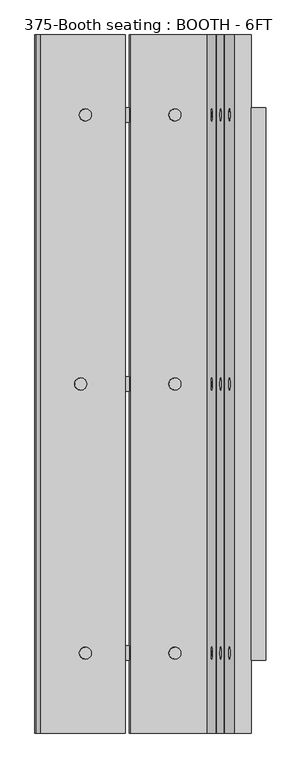
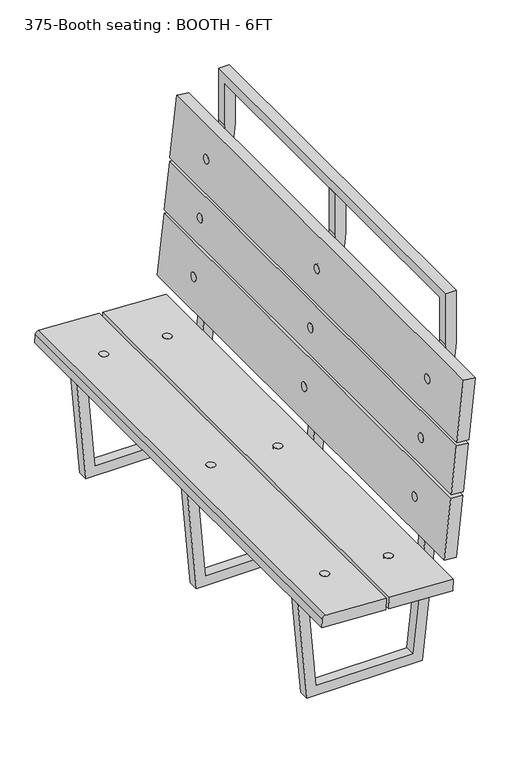
"""IFC4 building model written with IfcOpenShell, lengths in millimetres: furniture geometry, 375-Booth seating : BOOTH - 6FT."""

from ifc_helpers import new_model, si_unit, point, frame, frame_2d, origin, place, context, project, spatial, polyline, circle_curve, trimmed, segment, composite_curve, outline, extrude, faceted_brep, source, transform, mapped, element, save


def furniture_375_booth_seating_booth_6ft_eb83aa60(model_context):
    return source(origin(), model_context, "Body", "SolidModel", [
        extrude(outline(composite_curve([segment(trimmed(circle_curve(frame_2d((0.0, -15.875)), 15.875), [point((0.0, -31.75))], [point((0.0, 0.0))], False, "CARTESIAN"), True, "CONTINUOUS"), segment(trimmed(circle_curve(frame_2d((0.0, -15.875)), 15.875), [point((0.0, 0.0))], [point((0.0, -31.75))], False, "CARTESIAN"), True, "CONTINUOUS")], self_intersect=False)), frame((476.8022404, 688.975, 403.0070028), z_axis=(0.052335956242943765, 0.0, 0.9986295347545739), x_axis=(-0.9986295347545739, 0.0, 0.052335956242943765)), (0.0, 0.0, 1.0), 44.45),
        extrude(outline(composite_curve([segment(trimmed(circle_curve(frame_2d((-234.95, -15.875)), 15.875), [point((-234.95, -31.75))], [point((-234.95, 0.0))], False, "CARTESIAN"), True, "CONTINUOUS"), segment(trimmed(circle_curve(frame_2d((-234.95, -15.875)), 15.875), [point((-234.95, 0.0))], [point((-234.95, -31.75))], False, "CARTESIAN"), True, "CONTINUOUS")], self_intersect=False)), frame((476.8022404, 688.975, 403.0070028), z_axis=(0.052335956242943765, 0.0, 0.9986295347545739), x_axis=(-0.9986295347545739, 0.0, 0.052335956242943765)), (0.0, 0.0, 1.0), 44.45),
        extrude(outline(composite_curve([segment(trimmed(circle_curve(frame_2d((0.0, 1393.825)), 15.875), [point((0.0, 1377.95))], [point((0.0, 1409.7))], False, "CARTESIAN"), True, "CONTINUOUS"), segment(trimmed(circle_curve(frame_2d((0.0, 1393.825)), 15.875), [point((0.0, 1409.7))], [point((0.0, 1377.95))], False, "CARTESIAN"), True, "CONTINUOUS")], self_intersect=False)), frame((476.8022404, 688.975, 403.0070028), z_axis=(0.052335956242943765, 0.0, 0.9986295347545739), x_axis=(-0.9986295347545739, 0.0, 0.052335956242943765)), (0.0, 0.0, 1.0), 44.45),
        extrude(outline(composite_curve([segment(trimmed(circle_curve(frame_2d((-234.95, 1393.825)), 15.875), [point((-234.95, 1377.95))], [point((-234.95, 1409.7))], False, "CARTESIAN"), True, "CONTINUOUS"), segment(trimmed(circle_curve(frame_2d((-234.95, 1393.825)), 15.875), [point((-234.95, 1409.7))], [point((-234.95, 1377.95))], False, "CARTESIAN"), True, "CONTINUOUS")], self_intersect=False)), frame((476.8022404, 688.975, 403.0070028), z_axis=(0.052335956242943765, 0.0, 0.9986295347545739), x_axis=(-0.9986295347545739, 0.0, 0.052335956242943765)), (0.0, 0.0, 1.0), 44.45),
        extrude(outline(composite_curve([segment(trimmed(circle_curve(frame_2d((0.0, -15.875)), 15.875), [point((0.0, -31.75))], [point((0.0, 0.0))], False, "CARTESIAN"), True, "CONTINUOUS"), segment(trimmed(circle_curve(frame_2d((0.0, -15.875)), 15.875), [point((0.0, 0.0))], [point((0.0, -31.75))], False, "CARTESIAN"), True, "CONTINUOUS")], self_intersect=False)), frame((900.6975371, -720.725, 1069.1522612), z_axis=(-0.9945218953682735, 0.0, 0.10452846326765225), x_axis=(-0.10452846326765225, 0.0, -0.9945218953682735)), (0.0, 0.0, 1.0), 44.45),
        extrude(outline(composite_curve([segment(trimmed(circle_curve(frame_2d((222.2499999, -15.875)), 15.875), [point((222.2499999, -31.75))], [point((222.2499999, 0.0))], False, "CARTESIAN"), True, "CONTINUOUS"), segment(trimmed(circle_curve(frame_2d((222.2499999, -15.875)), 15.875), [point((222.2499999, 0.0))], [point((222.2499999, -31.75))], False, "CARTESIAN"), True, "CONTINUOUS")], self_intersect=False)), frame((900.6975371, -720.725, 1069.1522612), z_axis=(-0.9945218953682735, 0.0, 0.10452846326765225), x_axis=(-0.10452846326765225, 0.0, -0.9945218953682735)), (0.0, 0.0, 1.0), 44.45),
        extrude(outline(composite_curve([segment(trimmed(circle_curve(frame_2d((444.5, -15.875)), 15.875), [point((444.5, -31.75))], [point((444.5, 0.0))], False, "CARTESIAN"), True, "CONTINUOUS"), segment(trimmed(circle_curve(frame_2d((444.5, -15.875)), 15.875), [point((444.5, 0.0))], [point((444.5, -31.75))], False, "CARTESIAN"), True, "CONTINUOUS")], self_intersect=False)), frame((900.6975371, -720.725, 1069.1522612), z_axis=(-0.9945218953682735, 0.0, 0.10452846326765225), x_axis=(-0.10452846326765225, 0.0, -0.9945218953682735)), (0.0, 0.0, 1.0), 44.45),
        extrude(outline(composite_curve([segment(trimmed(circle_curve(frame_2d((0.0, -1425.575)), 15.875), [point((0.0, -1441.45))], [point((0.0, -1409.7))], False, "CARTESIAN"), True, "CONTINUOUS"), segment(trimmed(circle_curve(frame_2d((0.0, -1425.575)), 15.875), [point((0.0, -1409.7))], [point((0.0, -1441.45))], False, "CARTESIAN"), True, "CONTINUOUS")], self_intersect=False)), frame((900.6975371, -720.725, 1069.1522612), z_axis=(-0.9945218953682735, 0.0, 0.10452846326765225), x_axis=(-0.10452846326765225, 0.0, -0.9945218953682735)), (0.0, 0.0, 1.0), 44.45),
        extrude(outline(composite_curve([segment(trimmed(circle_curve(frame_2d((222.2499999, -1425.575)), 15.875), [point((222.2499999, -1441.45))], [point((222.2499999, -1409.7))], False, "CARTESIAN"), True, "CONTINUOUS"), segment(trimmed(circle_curve(frame_2d((222.2499999, -1425.575)), 15.875), [point((222.2499999, -1409.7))], [point((222.2499999, -1441.45))], False, "CARTESIAN"), True, "CONTINUOUS")], self_intersect=False)), frame((900.6975371, -720.725, 1069.1522612), z_axis=(-0.9945218953682735, 0.0, 0.10452846326765225), x_axis=(-0.10452846326765225, 0.0, -0.9945218953682735)), (0.0, 0.0, 1.0), 44.45),
        extrude(outline(composite_curve([segment(trimmed(circle_curve(frame_2d((444.5, -1425.575)), 15.875), [point((444.5, -1441.45))], [point((444.5, -1409.7))], False, "CARTESIAN"), True, "CONTINUOUS"), segment(trimmed(circle_curve(frame_2d((444.5, -1425.575)), 15.875), [point((444.5, -1409.7))], [point((444.5, -1441.45))], False, "CARTESIAN"), True, "CONTINUOUS")], self_intersect=False)), frame((900.6975371, -720.725, 1069.1522612), z_axis=(-0.9945218953682735, 0.0, 0.10452846326765225), x_axis=(-0.10452846326765225, 0.0, -0.9945218953682735)), (0.0, 0.0, 1.0), 44.45),
        extrude(outline(composite_curve([segment(trimmed(circle_curve(frame_2d((0.0, -15.875)), 15.875), [point((0.0, -31.75))], [point((0.0, 0.0))], False, "CARTESIAN"), True, "CONTINUOUS"), segment(trimmed(circle_curve(frame_2d((0.0, -15.875)), 15.875), [point((0.0, 0.0))], [point((0.0, -31.75))], False, "CARTESIAN"), True, "CONTINUOUS")], self_intersect=False)), frame((464.1196453, -15.875, 403.6716695), z_axis=(0.052335956242943765, 0.0, 0.9986295347545739), x_axis=(-0.9986295347545739, 0.0, 0.052335956242943765)), (0.0, 0.0, 1.0), 44.45),
        extrude(outline(composite_curve([segment(trimmed(circle_curve(frame_2d((-247.65, -15.875)), 15.875), [point((-247.65, -31.75))], [point((-247.65, 0.0))], False, "CARTESIAN"), True, "CONTINUOUS"), segment(trimmed(circle_curve(frame_2d((-247.65, -15.875)), 15.875), [point((-247.65, 0.0))], [point((-247.65, -31.75))], False, "CARTESIAN"), True, "CONTINUOUS")], self_intersect=False)), frame((464.1196453, -15.875, 403.6716695), z_axis=(0.052335956242943765, 0.0, 0.9986295347545739), x_axis=(-0.9986295347545739, 0.0, 0.052335956242943765)), (0.0, 0.0, 1.0), 44.45),
        extrude(outline(composite_curve([segment(trimmed(circle_curve(frame_2d((0.0, -15.875)), 15.875), [point((0.0, -31.75))], [point((0.0, 0.0))], False, "CARTESIAN"), True, "CONTINUOUS"), segment(trimmed(circle_curve(frame_2d((0.0, -15.875)), 15.875), [point((0.0, 0.0))], [point((0.0, -31.75))], False, "CARTESIAN"), True, "CONTINUOUS")], self_intersect=False)), frame((900.6975371, -15.875, 1069.1522612), z_axis=(-0.9945218953682735, 0.0, 0.10452846326765225), x_axis=(-0.10452846326765225, 0.0, -0.9945218953682735)), (0.0, 0.0, 1.0), 44.45),
        extrude(outline(composite_curve([segment(trimmed(circle_curve(frame_2d((222.2499999, -15.875)), 15.875), [point((222.2499999, -31.75))], [point((222.2499999, 0.0))], False, "CARTESIAN"), True, "CONTINUOUS"), segment(trimmed(circle_curve(frame_2d((222.2499999, -15.875)), 15.875), [point((222.2499999, 0.0))], [point((222.2499999, -31.75))], False, "CARTESIAN"), True, "CONTINUOUS")], self_intersect=False)), frame((900.6975371, -15.875, 1069.1522612), z_axis=(-0.9945218953682735, 0.0, 0.10452846326765225), x_axis=(-0.10452846326765225, 0.0, -0.9945218953682735)), (0.0, 0.0, 1.0), 44.45),
        extrude(outline(composite_curve([segment(trimmed(circle_curve(frame_2d((444.5, -15.875)), 15.875), [point((444.5, -31.75))], [point((444.5, 0.0))], False, "CARTESIAN"), True, "CONTINUOUS"), segment(trimmed(circle_curve(frame_2d((444.5, -15.875)), 15.875), [point((444.5, 0.0))], [point((444.5, -31.75))], False, "CARTESIAN"), True, "CONTINUOUS")], self_intersect=False)), frame((900.6975371, -15.875, 1069.1522612), z_axis=(-0.9945218953682735, 0.0, 0.10452846326765225), x_axis=(-0.10452846326765225, 0.0, -0.9945218953682735)), (0.0, 0.0, 1.0), 44.45),
        extrude(outline(polyline([(384.5625035, 828.7442542), (408.7701083, 366.8356381), (0.0, 402.5983885), (0.0, 826.6349718), (1193.8, 952.1084079), (1358.9, 952.1084079), (1358.9, 914.0084079), (1195.7967364, 914.0084079), (384.5625035, 828.7442542)]), holes=[polyline([(38.1, 437.5106063), (368.4284885, 408.6106083), (346.6192193, 824.7562543), (38.1, 792.3295777), (38.1, 437.5106063)])]), frame((0.0, -19.05, 0.0), z_axis=(0.0, 1.0, 0.0), x_axis=(0.0, 0.0, 1.0)), (0.0, 0.0, 1.0), 38.1),
        faceted_brep([(828.7442542, -685.8, 384.5625035), (914.0084079, -685.8, 1195.7967364), (914.0084079, -685.8, 1358.9), (952.1084079, -685.8, 1358.9), (952.1084079, -685.8, 1193.8), (826.6349718, -685.8, 0.0), (402.5983885, -685.8, 0.0), (366.8356381, -685.8, 408.7701083), (437.5106063, -685.8, 38.1), (792.3295777, -685.8, 38.1), (824.7562543, -685.8, 346.6192193), (408.6106083, -685.8, 368.4284885), (828.7442542, -723.9, 384.5625035), (366.8356381, -723.9, 408.7701083), (402.5983885, -723.9, 0.0), (826.6349718, -723.9, 0.0), (952.1084079, -723.9, 1193.8), (952.1084079, -723.9, 1397.0), (914.0084079, -723.9, 1397.0), (914.0084079, -723.9, 1195.7967364), (437.5106063, -723.9, 38.1), (408.6106083, -723.9, 368.4284885), (824.7562543, -723.9, 346.6192193), (792.3295777, -723.9, 38.1), (914.0084079, 685.8, 1358.9), (952.1084079, 685.8, 1358.9), (828.7442542, 723.9, 384.5625035), (914.0084079, 723.9, 1195.7967364), (914.0084079, 723.9, 1397.0), (952.1084079, 723.9, 1397.0), (952.1084079, 723.9, 1193.8), (826.6349718, 723.9, 0.0), (402.5983885, 723.9, 0.0), (366.8356381, 723.9, 408.7701083), (437.5106063, 723.9, 38.1), (792.3295777, 723.9, 38.1), (824.7562543, 723.9, 346.6192193), (408.6106083, 723.9, 368.4284885), (828.7442542, 685.8, 384.5625035), (366.8356381, 685.8, 408.7701083), (402.5983885, 685.8, 0.0), (826.6349718, 685.8, 0.0), (952.1084079, 685.8, 1193.8), (914.0084079, 685.8, 1195.7967364), (437.5106063, 685.8, 38.1), (408.6106083, 685.8, 368.4284885), (824.7562543, 685.8, 346.6192193), (792.3295777, 685.8, 38.1)], [[[0, 1, 2, 3, 4, 5, 6, 7], [8, 9, 10, 11]], [[12, 13, 14, 15, 16, 17, 18, 19], [20, 21, 22, 23]], [[5, 4, 16, 15]], [[1, 0, 12, 19]], [[0, 7, 13, 12]], [[7, 6, 14, 13]], [[6, 5, 15, 14]], [[8, 11, 21, 20]], [[11, 10, 22, 21]], [[10, 9, 23, 22]], [[9, 8, 20, 23]], [[2, 24, 25, 3]], [[26, 27, 28, 29, 30, 31, 32, 33], [34, 35, 36, 37]], [[38, 39, 40, 41, 42, 25, 24, 43], [44, 45, 46, 47]], [[26, 33, 39, 38]], [[33, 32, 40, 39]], [[32, 31, 41, 40]], [[34, 37, 45, 44]], [[37, 36, 46, 45]], [[36, 35, 47, 46]], [[35, 34, 44, 47]], [[31, 30, 42, 41]], [[27, 26, 38, 43]], [[17, 16, 4, 3, 25, 42, 30, 29]], [[18, 17, 29, 28]], [[19, 18, 28, 27, 43, 24, 2, 1]]]),
        extrude(outline(polyline([(0.0, -44.45), (0.0, 0.0), (1828.8, 0.0), (1828.8, -44.45), (0.0, -44.45)])), frame((841.955154, 914.4, 510.2558191), z_axis=(0.10452846326765272, 0.0, 0.9945218953682734), x_axis=(0.0, -1.0, 0.0)), (0.0, 0.0, 1.0), 234.95),
        extrude(outline(polyline([(0.0, -44.45), (0.0, 0.0), (1828.8, 0.0), (1828.8, -44.45), (0.0, -44.45)])), frame((867.8416279, 914.4, 756.5491664), z_axis=(0.10452846326765385, 0.0, 0.9945218953682733), x_axis=(0.0, -1.0, 0.0)), (0.0, 0.0, 1.0), 184.15),
        extrude(outline(polyline([(0.0, -44.45), (0.0, 0.0), (1828.8, 0.0), (1828.8, -44.45), (0.0, -44.45)])), frame((888.4180559, 914.4, 952.3208015), z_axis=(0.10452846326765004, 0.0, 0.9945218953682737), x_axis=(0.0, -1.0, 0.0)), (0.0, 0.0, 1.0), 234.95),
        extrude(outline(composite_curve([segment(polyline([(441.9125858, 583.7599832), (453.5442521, 361.8145691)]), True, "CONTINUOUS"), segment(trimmed(circle_curve(frame_2d((440.861657, 361.1499024)), 12.7), [point((453.5442521, 361.8145691))], [point((441.5263237, 348.4673073))], False, "CARTESIAN"), True, "CONTINUOUS"), segment(polyline([(441.5263237, 348.4673073), (409.8198359, 346.8056407), (397.4995564, 581.8905778), (441.9125858, 583.7599832)]), True, "CONTINUOUS")], self_intersect=False)), frame((0.0, -914.4, 0.0), z_axis=(0.0, 1.0, 0.0), x_axis=(0.0, 0.0, 1.0)), (0.0, 0.0, 1.0), 1828.8),
        extrude(outline(polyline([(0.0, -234.95), (0.0, 0.0), (1828.8, 0.0), (1828.8, -234.95), (0.0, -234.95)])), frame((828.7442542, 914.4, 384.5625035), z_axis=(0.05233595624294369, 0.0, 0.9986295347545739), x_axis=(0.0, -1.0, 0.0)), (0.0, 0.0, 1.0), 44.45),
    ])


if __name__ == "__main__":
    model = new_model("IFC4")
    model_context = context("Model", 3, world=origin())
    ifc_project = project(units=[si_unit("LENGTHUNIT", "METRE", prefix="MILLI")], contexts=[model_context])
    site = spatial("IfcSite", under=ifc_project)
    building = spatial("IfcBuilding", under=site)
    placement = place(None, origin())
    furniture_375_booth_seating_booth_6ft_shape = furniture_375_booth_seating_booth_6ft_eb83aa60(model_context)
    element("IfcFurniture", 1, ObjectType="375-Booth seating : BOOTH - 6FT", at=placement, inside=building, context=model_context, shape_type="MappedRepresentation", body=[
        mapped(furniture_375_booth_seating_booth_6ft_shape, transform((0.0, 0.0, 0.0), x_axis=(1.0, 0.0, 0.0), y_axis=(0.0, 1.0, 0.0), z_axis=(0.0, 0.0, 1.0))),
    ])
    save(model, "model.ifc")

# Revit data of these elements
# Type "375-Booth seating : BOOTH - 6FT"
#   tube dim [instance default] = 0' - 1 1/2"
#   seat angle = 3.00°
#   radius of plug = 0' - 0 5/8"
#   plank width_2 = 0' - 7 1/4"
#   plank width_1 = 0' - 9 1/4"
#   plank depth = 0' - 1 3/4"
#   inset = 0' - 9"
#   gap = 0' - 0 1/2"
#   DEPTH = 6' - 0"
#   Seating Count = 3
#   middle support visibility = yes
#   Right Bench Visible [instance default] = yes
#   Left Bench Visible [instance default] = yes
#   Material_1 = WOOD-OAKFIRE
#   Material 2 = 1 1/2" SQUARE TUBE STEEL\n- WELDED MITER JOINTS GROUND SMOOTH\n- CLEAR COAT
#   Assembly Code = ""
# Element 1 (IfcFurniture, "375-Booth seating : BOOTH - 6FT")
#   Materials on its faces: "1 1/2\" SQUARE TUBE STEEL\n- WELDED MITER JOINTS GROUND SMOOTH\n- CLEAR COAT", "1 1/4\" WOOD PLUG\n(SLIGHTLY DARKER OR STAINED WOOD) - GAL. HEX HEAD THRU BOLT", "WOOD-OAKFIRE"
# Materials
#   "WOOD-OAKFIRE": class "Wood", colour RGB 198 202 183, transparency 0, Description = "Generic wood", Cost = 0
#   "1 1/2\" SQUARE TUBE STEEL\n- WELDED MITER JOINTS GROUND SMOOTH\n- CLEAR COAT": class "Metal", colour RGB 147 147 147, transparency 0, Cost = 0
#   "1 1/4\" WOOD PLUG\n(SLIGHTLY DARKER OR STAINED WOOD) - GAL. HEX HEAD THRU BOLT": class "Generic", colour RGB 192 192 192, transparency 0, Cost = 0
